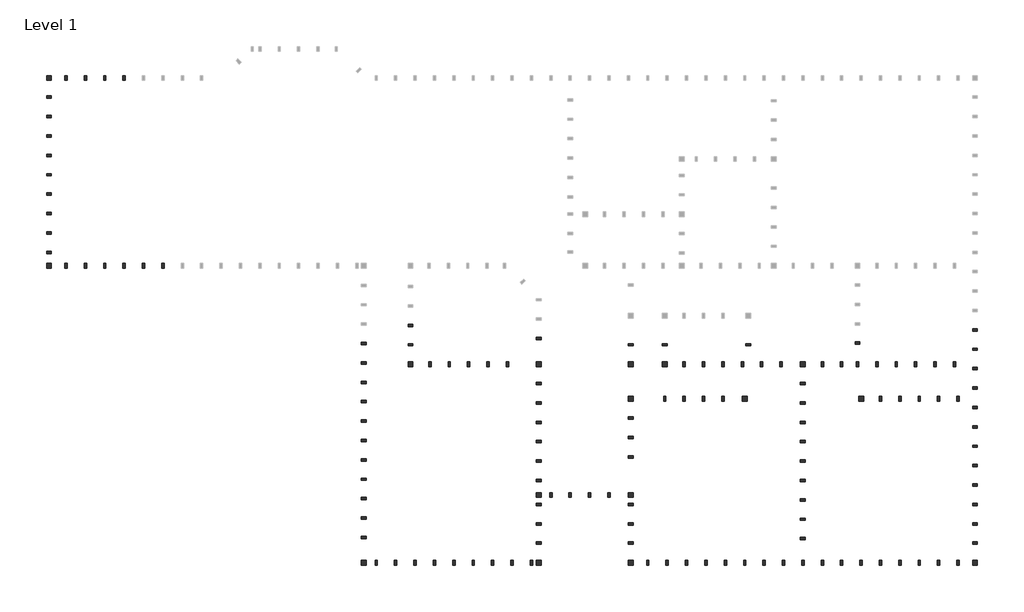
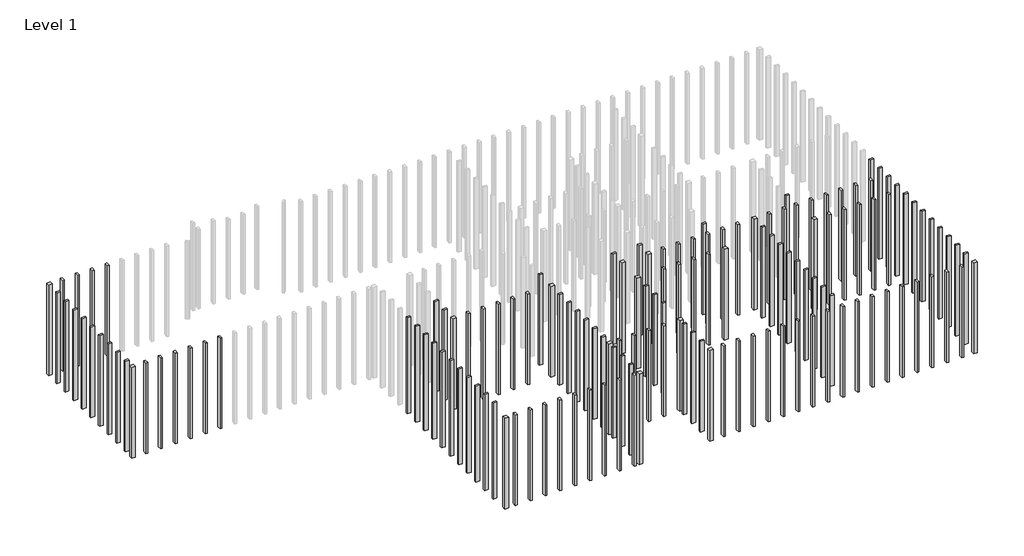
# One storey, part 1 of 2: 147 columns.
"""IFC4 building model written with IfcOpenShell, lengths in millimetres."""

import ifcopenshell
import ifcopenshell.guid

model = None  # the IFC model being written
_history = None  # IfcOwnerHistory: only IFC2X3 demands one
_inside = {}  # id of a spatial element -> (the spatial element, [elements in it])
_under = {}  # id of a project, library or spatial element -> (it, [spatial elements below it])
_declared = {}  # id of a project -> (the project, [libraries it declares])
_typed = {}  # id of a type object -> (the type object, [elements of that type])
_made_of = {}  # id of a material, layer set ... -> (it, [elements and type objects made of it])


def new_model(schema):
    """Start an empty IFC model of exactly this schema.

    Asked for "IFC4X3", IfcOpenShell would pick the latest addendum, in which some entities
    have other attributes; the version numbers below select the first issue.
    IFC2X3 requires an IfcOwnerHistory on every rooted entity: one is made here for all.
    """
    global model, _history
    if schema == "IFC4X3":
        model = ifcopenshell.file(schema_version=(4, 3, 0, 0))
    else:
        model = ifcopenshell.file(schema=schema)
    _inside.clear()
    _under.clear()
    _declared.clear()
    _typed.clear()
    _made_of.clear()
    _history = None
    if model.schema == "IFC2X3":
        org = make("IfcOrganization", Name="unknown")
        user = make(
            "IfcPersonAndOrganization",
            ThePerson=make("IfcPerson", FamilyName="unknown"),
            TheOrganization=org,
        )
        app = make(
            "IfcApplication",
            ApplicationDeveloper=org,
            Version="unknown",
            ApplicationFullName="unknown",
            ApplicationIdentifier="unknown",
        )
        _history = make(
            "IfcOwnerHistory",
            OwningUser=user,
            OwningApplication=app,
            ChangeAction="ADDED",
            CreationDate=0,
        )
    return model


def make(cls, **values):
    """One entity of the class cls with the attributes given. An attribute that is None is left unset."""
    return model.create_entity(
        cls, **{name: value for name, value in values.items() if value is not None}
    )


def rooted(cls, **values):
    """An entity with a GlobalId (a new one), such as an element, a storey or a relation."""
    return make(cls, GlobalId=ifcopenshell.guid.new(), OwnerHistory=_history, **values)


def si_unit(unit_type, name, prefix=None):
    """IfcSIUnit, for example si_unit("LENGTHUNIT", "METRE", prefix="MILLI")."""
    return make("IfcSIUnit", UnitType=unit_type, Prefix=prefix, Name=name)


def assignment(units):
    """IfcUnitAssignment: the units of a project."""
    return None if units is None else make("IfcUnitAssignment", Units=units)


def point(xyz):
    """IfcCartesianPoint."""
    return None if xyz is None else make("IfcCartesianPoint", Coordinates=xyz)


def direction(xyz):
    """IfcDirection."""
    return None if xyz is None else make("IfcDirection", DirectionRatios=xyz)


def frame(location, z_axis=None, x_axis=None):
    """IfcAxis2Placement3D, a coordinate frame: its origin and axes. An axis left out is left unset."""
    return make(
        "IfcAxis2Placement3D",
        Location=point(location),
        Axis=direction(z_axis),
        RefDirection=direction(x_axis),
    )


def origin():
    """The frame at (0, 0, 0) with its axes left unset."""
    return frame((0.0, 0.0, 0.0))


def origin_with_axes():
    """The frame at (0, 0, 0) with the z axis (0, 0, 1) and the x axis (1, 0, 0) written out."""
    return frame((0.0, 0.0, 0.0), z_axis=(0.0, 0.0, 1.0), x_axis=(1.0, 0.0, 0.0))


def place(relative_to, where):
    """IfcLocalPlacement: puts the frame where relative to a parent placement (None: the world)."""
    return make(
        "IfcLocalPlacement", PlacementRelTo=relative_to, RelativePlacement=where
    )


def context(
    kind, dimensions, precision=None, world=None, true_north=None, identifier=None
):
    """IfcGeometricRepresentationContext, for example the 3D "Model" context."""
    return make(
        "IfcGeometricRepresentationContext",
        ContextIdentifier=identifier,
        ContextType=kind,
        CoordinateSpaceDimension=dimensions,
        Precision=precision,
        WorldCoordinateSystem=world,
        TrueNorth=true_north,
    )


def project(units=None, contexts=None):
    """IfcProject with its units and contexts."""
    return rooted(
        "IfcProject",
        Name="project",
        RepresentationContexts=contexts,
        UnitsInContext=assignment(units),
    )


def spatial(cls, under=None, at=None, **own):
    """A site, building, storey or space (cls), placed at a placement, below another one or the project."""
    s = rooted(cls, ObjectPlacement=at, **own)
    if under is not None:
        _under.setdefault(under.id(), (under, []))[1].append(s)
    return s


def polyline(points):
    """IfcPolyline through the points."""
    return make("IfcPolyline", Points=[point(p) for p in points])


def outline(outer, holes=None, kind="AREA"):
    """IfcArbitraryClosedProfileDef: a profile drawn as a closed curve; with holes, ...WithVoids."""
    if holes is None:
        return make("IfcArbitraryClosedProfileDef", ProfileType=kind, OuterCurve=outer)
    return make(
        "IfcArbitraryProfileDefWithVoids",
        ProfileType=kind,
        OuterCurve=outer,
        InnerCurves=holes,
    )


def extrude(swept, where, along, depth):
    """IfcExtrudedAreaSolid: the profile swept, set in the frame where, extruded along a direction by depth."""
    return make(
        "IfcExtrudedAreaSolid",
        SweptArea=swept,
        Position=where,
        ExtrudedDirection=direction(along),
        Depth=depth,
    )


def shape(context_of_items, identifier, shape_type, items):
    """IfcShapeRepresentation: the items that make up one representation, for example the "Body"."""
    return make(
        "IfcShapeRepresentation",
        ContextOfItems=context_of_items,
        RepresentationIdentifier=identifier,
        RepresentationType=shape_type,
        Items=items,
    )


def source(mapping_origin, context_of_items, identifier, shape_type, items):
    """IfcRepresentationMap: a shape defined once, which mapped items show again and again."""
    return make(
        "IfcRepresentationMap",
        MappingOrigin=mapping_origin,
        MappedRepresentation=shape(context_of_items, identifier, shape_type, items),
    )


def transform(
    local_origin,
    x_axis=None,
    y_axis=None,
    z_axis=None,
    scale=None,
    scale2=None,
    scale3=None,
    uniform=True,
):
    """IfcCartesianTransformationOperator3D, or its non-uniform kind. x_axis, y_axis, z_axis: its Axis1, 2, 3."""
    if uniform:
        return make(
            "IfcCartesianTransformationOperator3D",
            Axis1=direction(x_axis),
            Axis2=direction(y_axis),
            LocalOrigin=point(local_origin),
            Scale=scale,
            Axis3=direction(z_axis),
        )
    return make(
        "IfcCartesianTransformationOperator3DnonUniform",
        Axis1=direction(x_axis),
        Axis2=direction(y_axis),
        LocalOrigin=point(local_origin),
        Scale=scale,
        Axis3=direction(z_axis),
        Scale2=scale2,
        Scale3=scale3,
    )


def mapped(mapping_source, mapping_target):
    """IfcMappedItem: shows the shape of a source again, moved by a transform."""
    return make(
        "IfcMappedItem", MappingSource=mapping_source, MappingTarget=mapping_target
    )


def made_of(thing, what):
    """Note that an element or type object is made of a material, layer set ...; save() writes the relation."""
    if what is not None:
        _made_of.setdefault(what.id(), (what, []))[1].append(thing)
    return thing


def element(
    cls,
    number,
    at=None,
    inside=None,
    cuts=None,
    type_object=None,
    material=None,
    context=None,
    identifier="Body",
    shape_type=None,
    held_by="IfcProductDefinitionShape",
    body=None,
    shapes=None,
    **own,
):
    """One element of the class cls, such as IfcWall. Its Tag is "e" and its number.

    at: its placement. inside: the storey or other place that contains it. cuts: it is an
    opening in that element (IfcRelVoidsElement). A single representation is given by context,
    identifier, shape_type and body (its items); several are given by shapes. held_by: the class
    of the entity that holds the representations. save() writes the other relations.
    """
    e = rooted(cls, Tag="e%d" % number, ObjectPlacement=at, **own)
    if body is not None:
        shapes = [shape(context, identifier, shape_type, body)]
    if shapes is not None:
        e.Representation = make(held_by, Representations=shapes)
    if inside is not None:
        _inside.setdefault(inside.id(), (inside, []))[1].append(e)
    if cuts is not None:
        rooted(
            "IfcRelVoidsElement", RelatingBuildingElement=cuts, RelatedOpeningElement=e
        )
    if type_object is not None:
        _typed.setdefault(type_object.id(), (type_object, []))[1].append(e)
    return made_of(e, material)


def aggregate(whole, parts):
    """IfcRelAggregates: a whole, such as a stair, and the parts it consists of."""
    return rooted("IfcRelAggregates", RelatingObject=whole, RelatedObjects=parts)


def save(model, path):
    """Write the relations noted so far, then the file.

    IfcRelAggregates (storeys below a building ...), IfcRelContainedInSpatialStructure (elements
    in a storey), IfcRelDefinesByType, IfcRelAssociatesMaterial and IfcRelDeclares: one each for
    every whole, place, type object, material and project.
    """
    for whole, parts in _under.values():
        aggregate(whole, parts)
    for where, things in _inside.values():
        rooted(
            "IfcRelContainedInSpatialStructure",
            RelatedElements=things,
            RelatingStructure=where,
        )
    for kind, things in _typed.values():
        rooted("IfcRelDefinesByType", RelatedObjects=things, RelatingType=kind)
    for what, things in _made_of.values():
        rooted("IfcRelAssociatesMaterial", RelatedObjects=things, RelatingMaterial=what)
    for by, libraries in _declared.values():
        rooted("IfcRelDeclares", RelatingContext=by, RelatedDefinitions=libraries)
    model.write(path)


def timber_column_65e54e3c(model_context):
    return source(origin(), model_context, "Body", "SweptSolid", [
        extrude(outline(polyline([(25.4, 50.8), (25.4, -50.8), (-25.4, -50.8), (-25.4, 50.8), (25.4, 50.8)])), frame((0.0, 0.0, 50.8), z_axis=(0.0, 0.0, 1.0), x_axis=(1.0, 0.0, 0.0)), (0.0, 0.0, 1.0), 2616.2),
    ])


def timber_column_b7e6a7b9(model_context):
    return source(origin(), model_context, "Body", "SweptSolid", [
        extrude(outline(polyline([(50.8, 50.8), (50.8, -50.8), (-50.8, -50.8), (-50.8, 50.8), (50.8, 50.8)])), frame((0.0, 0.0, 50.8), z_axis=(0.0, 0.0, 1.0), x_axis=(1.0, 0.0, 0.0)), (0.0, 0.0, 1.0), 2616.2),
    ])


def timber_column_c014de30(model_context):
    return source(origin(), model_context, "Body", "SweptSolid", [
        extrude(outline(polyline([(25.4, -50.8), (-25.4, -50.8), (-25.4, 50.8), (25.4, 50.8), (25.4, -50.8)])), frame((0.0, 0.0, 50.8), z_axis=(0.0, 0.0, 1.0), x_axis=(1.0, 0.0, 0.0)), (0.0, 0.0, 1.0), 2616.2),
    ])


def timber_column_7e99ce9a(model_context):
    return source(origin(), model_context, "Body", "SweptSolid", [
        extrude(outline(polyline([(25.4, 50.8), (25.4, -50.8), (-25.4, -50.8), (-25.4, 50.8), (25.4, 50.8)])), origin_with_axes(), (0.0, 0.0, 1.0), 2768.6),
    ])


model = new_model("IFC4")

# Units and contexts
model_context = context("Model", 3, world=origin())
ifc_project = project(units=[si_unit("LENGTHUNIT", "METRE", prefix="MILLI")], contexts=[model_context])

# Site, building, storey
site = spatial("IfcSite", under=ifc_project)
building = spatial("IfcBuilding", under=site)
storey = spatial("IfcBuildingStorey", under=building, Name="Level 1", Elevation=0.0)

# Columns
placement = place(None, origin())
timber_column_shape = timber_column_65e54e3c(model_context)
element("IfcColumn", 1, ObjectType="Timber-Column", at=placement, inside=storey, context=model_context, shape_type="MappedRepresentation", body=[
    mapped(timber_column_shape, transform((-17394.814829, 5156.9284114, 0.0), x_axis=(1.0, 0.0, 0.0), y_axis=(0.0, 1.0, 0.0), z_axis=(0.0, 0.0, 1.0))),
])
element("IfcColumn", 2, ObjectType="Timber-Column", at=placement, inside=storey, context=model_context, shape_type="MappedRepresentation", body=[
    mapped(timber_column_shape, transform((-16988.414829, 5156.9284114, 0.0), x_axis=(1.0, 0.0, 0.0), y_axis=(0.0, 1.0, 0.0), z_axis=(0.0, 0.0, 1.0))),
])
element("IfcColumn", 3, ObjectType="Timber-Column", at=placement, inside=storey, context=model_context, shape_type="MappedRepresentation", body=[
    mapped(timber_column_shape, transform((-16582.014829, 5156.9284114, 0.0), x_axis=(1.0, 0.0, 0.0), y_axis=(0.0, 1.0, 0.0), z_axis=(0.0, 0.0, 1.0))),
])
element("IfcColumn", 4, ObjectType="Timber-Column", at=placement, inside=storey, context=model_context, shape_type="MappedRepresentation", body=[
    mapped(timber_column_shape, transform((-16175.614829, 5156.9284114, 0.0), x_axis=(1.0, 0.0, 0.0), y_axis=(0.0, 1.0, 0.0), z_axis=(0.0, 0.0, 1.0))),
])
element("IfcColumn", 5, ObjectType="Timber-Column", at=placement, inside=storey, context=model_context, shape_type="MappedRepresentation", body=[
    mapped(timber_column_shape, transform((1299.585171, -5003.0715886, 0.0), x_axis=(1.0, 0.0, 0.0), y_axis=(0.0, 1.0, 0.0), z_axis=(0.0, 0.0, 1.0))),
])
element("IfcColumn", 6, ObjectType="Timber-Column", at=placement, inside=storey, context=model_context, shape_type="MappedRepresentation", body=[
    mapped(timber_column_shape, transform((893.185171, -5003.0715886, 0.0), x_axis=(1.0, 0.0, 0.0), y_axis=(0.0, 1.0, 0.0), z_axis=(0.0, 0.0, 1.0))),
])
element("IfcColumn", 7, ObjectType="Timber-Column", at=placement, inside=storey, context=model_context, shape_type="MappedRepresentation", body=[
    mapped(timber_column_shape, transform((486.785171, -5003.0715886, 0.0), x_axis=(1.0, 0.0, 0.0), y_axis=(0.0, 1.0, 0.0), z_axis=(0.0, 0.0, 1.0))),
])
element("IfcColumn", 8, ObjectType="Timber-Column", at=placement, inside=storey, context=model_context, shape_type="MappedRepresentation", body=[
    mapped(timber_column_shape, transform((80.385171, -5003.0715886, 0.0), x_axis=(1.0, 0.0, 0.0), y_axis=(0.0, 1.0, 0.0), z_axis=(0.0, 0.0, 1.0))),
])
element("IfcColumn", 9, ObjectType="Timber-Column", at=placement, inside=storey, context=model_context, shape_type="MappedRepresentation", body=[
    mapped(timber_column_shape, transform((-326.014829, -5003.0715886, 0.0), x_axis=(1.0, 0.0, 0.0), y_axis=(0.0, 1.0, 0.0), z_axis=(0.0, 0.0, 1.0))),
])
element("IfcColumn", 10, ObjectType="Timber-Column", at=placement, inside=storey, context=model_context, shape_type="MappedRepresentation", body=[
    mapped(timber_column_shape, transform((-732.414829, -5003.0715886, 0.0), x_axis=(1.0, 0.0, 0.0), y_axis=(0.0, 1.0, 0.0), z_axis=(0.0, 0.0, 1.0))),
])
element("IfcColumn", 11, ObjectType="Timber-Column", at=placement, inside=storey, context=model_context, shape_type="MappedRepresentation", body=[
    mapped(timber_column_shape, transform((-1138.814829, -5003.0715886, 0.0), x_axis=(1.0, 0.0, 0.0), y_axis=(0.0, 1.0, 0.0), z_axis=(0.0, 0.0, 1.0))),
])
element("IfcColumn", 12, ObjectType="Timber-Column", at=placement, inside=storey, context=model_context, shape_type="MappedRepresentation", body=[
    mapped(timber_column_shape, transform((-1545.214829, -5003.0715886, 0.0), x_axis=(1.0, 0.0, 0.0), y_axis=(0.0, 1.0, 0.0), z_axis=(0.0, 0.0, 1.0))),
])
element("IfcColumn", 13, ObjectType="Timber-Column", at=placement, inside=storey, context=model_context, shape_type="MappedRepresentation", body=[
    mapped(timber_column_shape, transform((-1951.614829, -5003.0715886, 0.0), x_axis=(1.0, 0.0, 0.0), y_axis=(0.0, 1.0, 0.0), z_axis=(0.0, 0.0, 1.0))),
])
element("IfcColumn", 14, ObjectType="Timber-Column", at=placement, inside=storey, context=model_context, shape_type="MappedRepresentation", body=[
    mapped(timber_column_shape, transform((-2358.014829, -5003.0715886, 0.0), x_axis=(1.0, 0.0, 0.0), y_axis=(0.0, 1.0, 0.0), z_axis=(0.0, 0.0, 1.0))),
])
element("IfcColumn", 15, ObjectType="Timber-Column", at=placement, inside=storey, context=model_context, shape_type="MappedRepresentation", body=[
    mapped(timber_column_shape, transform((-2764.414829, -5003.0715886, 0.0), x_axis=(1.0, 0.0, 0.0), y_axis=(0.0, 1.0, 0.0), z_axis=(0.0, 0.0, 1.0))),
])
element("IfcColumn", 16, ObjectType="Timber-Column", at=placement, inside=storey, context=model_context, shape_type="MappedRepresentation", body=[
    mapped(timber_column_shape, transform((-3170.814829, -5003.0715886, 0.0), x_axis=(1.0, 0.0, 0.0), y_axis=(0.0, 1.0, 0.0), z_axis=(0.0, 0.0, 1.0))),
])
element("IfcColumn", 17, ObjectType="Timber-Column", at=placement, inside=storey, context=model_context, shape_type="MappedRepresentation", body=[
    mapped(timber_column_shape, transform((-3577.214829, -5003.0715886, 0.0), x_axis=(1.0, 0.0, 0.0), y_axis=(0.0, 1.0, 0.0), z_axis=(0.0, 0.0, 1.0))),
])
element("IfcColumn", 18, ObjectType="Timber-Column", at=placement, inside=storey, context=model_context, shape_type="MappedRepresentation", body=[
    mapped(timber_column_shape, transform((-3983.614829, -5003.0715886, 0.0), x_axis=(1.0, 0.0, 0.0), y_axis=(0.0, 1.0, 0.0), z_axis=(0.0, 0.0, 1.0))),
])
element("IfcColumn", 19, ObjectType="Timber-Column", at=placement, inside=storey, context=model_context, shape_type="MappedRepresentation", body=[
    mapped(timber_column_shape, transform((-4390.014829, -5003.0715886, 0.0), x_axis=(1.0, 0.0, 0.0), y_axis=(0.0, 1.0, 0.0), z_axis=(0.0, 0.0, 1.0))),
])
element("IfcColumn", 20, ObjectType="Timber-Column", at=placement, inside=storey, context=model_context, shape_type="MappedRepresentation", body=[
    mapped(timber_column_shape, transform((-4796.414829, -5003.0715886, 0.0), x_axis=(1.0, 0.0, 0.0), y_axis=(0.0, 1.0, 0.0), z_axis=(0.0, 0.0, 1.0))),
])
element("IfcColumn", 21, ObjectType="Timber-Column", at=placement, inside=storey, context=model_context, shape_type="MappedRepresentation", body=[
    mapped(timber_column_shape, transform((-5202.814829, -5003.0715886, 0.0), x_axis=(1.0, 0.0, 0.0), y_axis=(0.0, 1.0, 0.0), z_axis=(0.0, 0.0, 1.0))),
])
element("IfcColumn", 22, ObjectType="Timber-Column", at=placement, inside=storey, context=model_context, shape_type="MappedRepresentation", body=[
    mapped(timber_column_shape, transform((-6015.614829, -3580.6715886, 0.0), x_axis=(1.0, 0.0, 0.0), y_axis=(0.0, 1.0, 0.0), z_axis=(0.0, 0.0, 1.0))),
])
element("IfcColumn", 23, ObjectType="Timber-Column", at=placement, inside=storey, context=model_context, shape_type="MappedRepresentation", body=[
    mapped(timber_column_shape, transform((-6422.014829, -3580.6715886, 0.0), x_axis=(1.0, 0.0, 0.0), y_axis=(0.0, 1.0, 0.0), z_axis=(0.0, 0.0, 1.0))),
])
element("IfcColumn", 24, ObjectType="Timber-Column", at=placement, inside=storey, context=model_context, shape_type="MappedRepresentation", body=[
    mapped(timber_column_shape, transform((-6828.414829, -3580.6715886, 0.0), x_axis=(1.0, 0.0, 0.0), y_axis=(0.0, 1.0, 0.0), z_axis=(0.0, 0.0, 1.0))),
])
element("IfcColumn", 25, ObjectType="Timber-Column", at=placement, inside=storey, context=model_context, shape_type="MappedRepresentation", body=[
    mapped(timber_column_shape, transform((-7234.814829, -3580.6715886, 0.0), x_axis=(1.0, 0.0, 0.0), y_axis=(0.0, 1.0, 0.0), z_axis=(0.0, 0.0, 1.0))),
])
element("IfcColumn", 26, ObjectType="Timber-Column", at=placement, inside=storey, context=model_context, shape_type="MappedRepresentation", body=[
    mapped(timber_column_shape, transform((-7641.214829, -5003.0715886, 0.0), x_axis=(1.0, 0.0, 0.0), y_axis=(0.0, 1.0, 0.0), z_axis=(0.0, 0.0, 1.0))),
])
element("IfcColumn", 27, ObjectType="Timber-Column", at=placement, inside=storey, context=model_context, shape_type="MappedRepresentation", body=[
    mapped(timber_column_shape, transform((-8047.614829, -5003.0715886, 0.0), x_axis=(1.0, 0.0, 0.0), y_axis=(0.0, 1.0, 0.0), z_axis=(0.0, 0.0, 1.0))),
])
element("IfcColumn", 28, ObjectType="Timber-Column", at=placement, inside=storey, context=model_context, shape_type="MappedRepresentation", body=[
    mapped(timber_column_shape, transform((-8454.014829, -5003.0715886, 0.0), x_axis=(1.0, 0.0, 0.0), y_axis=(0.0, 1.0, 0.0), z_axis=(0.0, 0.0, 1.0))),
])
element("IfcColumn", 29, ObjectType="Timber-Column", at=placement, inside=storey, context=model_context, shape_type="MappedRepresentation", body=[
    mapped(timber_column_shape, transform((-8860.414829, -5003.0715886, 0.0), x_axis=(1.0, 0.0, 0.0), y_axis=(0.0, 1.0, 0.0), z_axis=(0.0, 0.0, 1.0))),
])
element("IfcColumn", 30, ObjectType="Timber-Column", at=placement, inside=storey, context=model_context, shape_type="MappedRepresentation", body=[
    mapped(timber_column_shape, transform((-9266.814829, -5003.0715886, 0.0), x_axis=(1.0, 0.0, 0.0), y_axis=(0.0, 1.0, 0.0), z_axis=(0.0, 0.0, 1.0))),
])
element("IfcColumn", 31, ObjectType="Timber-Column", at=placement, inside=storey, context=model_context, shape_type="MappedRepresentation", body=[
    mapped(timber_column_shape, transform((-9673.214829, -5003.0715886, 0.0), x_axis=(1.0, 0.0, 0.0), y_axis=(0.0, 1.0, 0.0), z_axis=(0.0, 0.0, 1.0))),
])
element("IfcColumn", 32, ObjectType="Timber-Column", at=placement, inside=storey, context=model_context, shape_type="MappedRepresentation", body=[
    mapped(timber_column_shape, transform((-10079.614829, -5003.0715886, 0.0), x_axis=(1.0, 0.0, 0.0), y_axis=(0.0, 1.0, 0.0), z_axis=(0.0, 0.0, 1.0))),
])
element("IfcColumn", 33, ObjectType="Timber-Column", at=placement, inside=storey, context=model_context, shape_type="MappedRepresentation", body=[
    mapped(timber_column_shape, transform((-10486.014829, -5003.0715886, 0.0), x_axis=(1.0, 0.0, 0.0), y_axis=(0.0, 1.0, 0.0), z_axis=(0.0, 0.0, 1.0))),
])
element("IfcColumn", 34, ObjectType="Timber-Column", at=placement, inside=storey, context=model_context, shape_type="MappedRepresentation", body=[
    mapped(timber_column_shape, transform((-10892.414829, -5003.0715886, 0.0), x_axis=(1.0, 0.0, 0.0), y_axis=(0.0, 1.0, 0.0), z_axis=(0.0, 0.0, 1.0))),
])
element("IfcColumn", 35, ObjectType="Timber-Column", at=placement, inside=storey, context=model_context, shape_type="MappedRepresentation", body=[
    mapped(timber_column_shape, transform((-15362.814829, 1226.2784114, 0.0), x_axis=(1.0, 0.0, 0.0), y_axis=(0.0, 1.0, 0.0), z_axis=(0.0, 0.0, 1.0))),
])
element("IfcColumn", 36, ObjectType="Timber-Column", at=placement, inside=storey, context=model_context, shape_type="MappedRepresentation", body=[
    mapped(timber_column_shape, transform((-15769.214829, 1226.2784114, 0.0), x_axis=(1.0, 0.0, 0.0), y_axis=(0.0, 1.0, 0.0), z_axis=(0.0, 0.0, 1.0))),
])
element("IfcColumn", 37, ObjectType="Timber-Column", at=placement, inside=storey, context=model_context, shape_type="MappedRepresentation", body=[
    mapped(timber_column_shape, transform((-16175.614829, 1226.2784114, 0.0), x_axis=(1.0, 0.0, 0.0), y_axis=(0.0, 1.0, 0.0), z_axis=(0.0, 0.0, 1.0))),
])
element("IfcColumn", 38, ObjectType="Timber-Column", at=placement, inside=storey, context=model_context, shape_type="MappedRepresentation", body=[
    mapped(timber_column_shape, transform((-16582.014829, 1226.2784114, 0.0), x_axis=(1.0, 0.0, 0.0), y_axis=(0.0, 1.0, 0.0), z_axis=(0.0, 0.0, 1.0))),
])
element("IfcColumn", 39, ObjectType="Timber-Column", at=placement, inside=storey, context=model_context, shape_type="MappedRepresentation", body=[
    mapped(timber_column_shape, transform((-16988.414829, 1226.2784114, 0.0), x_axis=(1.0, 0.0, 0.0), y_axis=(0.0, 1.0, 0.0), z_axis=(0.0, 0.0, 1.0))),
])
element("IfcColumn", 40, ObjectType="Timber-Column", at=placement, inside=storey, context=model_context, shape_type="MappedRepresentation", body=[
    mapped(timber_column_shape, transform((-17394.814829, 1226.2784114, 0.0), x_axis=(1.0, 0.0, 0.0), y_axis=(0.0, 1.0, 0.0), z_axis=(0.0, 0.0, 1.0))),
])
element("IfcColumn", 41, ObjectType="Timber-Column", at=placement, inside=storey, context=model_context, shape_type="MappedRepresentation", body=[
    mapped(timber_column_shape, transform((-17750.414829, 4756.8784114, 0.0), x_axis=(0.0, 1.0, 0.0), y_axis=(-1.0, 0.0, 0.0), z_axis=(0.0, 0.0, 1.0))),
])
element("IfcColumn", 42, ObjectType="Timber-Column", at=placement, inside=storey, context=model_context, shape_type="MappedRepresentation", body=[
    mapped(timber_column_shape, transform((-17750.414829, 4350.4784114, 0.0), x_axis=(0.0, 1.0, 0.0), y_axis=(-1.0, 0.0, 0.0), z_axis=(0.0, 0.0, 1.0))),
])
element("IfcColumn", 43, ObjectType="Timber-Column", at=placement, inside=storey, context=model_context, shape_type="MappedRepresentation", body=[
    mapped(timber_column_shape, transform((-17750.414829, 3944.0784114, 0.0), x_axis=(0.0, 1.0, 0.0), y_axis=(-1.0, 0.0, 0.0), z_axis=(0.0, 0.0, 1.0))),
])
element("IfcColumn", 44, ObjectType="Timber-Column", at=placement, inside=storey, context=model_context, shape_type="MappedRepresentation", body=[
    mapped(timber_column_shape, transform((-17750.414829, 3537.6784114, 0.0), x_axis=(0.0, 1.0, 0.0), y_axis=(-1.0, 0.0, 0.0), z_axis=(0.0, 0.0, 1.0))),
])
element("IfcColumn", 45, ObjectType="Timber-Column", at=placement, inside=storey, context=model_context, shape_type="MappedRepresentation", body=[
    mapped(timber_column_shape, transform((-17750.414829, 3131.2784114, 0.0), x_axis=(0.0, 1.0, 0.0), y_axis=(-1.0, 0.0, 0.0), z_axis=(0.0, 0.0, 1.0))),
])
element("IfcColumn", 46, ObjectType="Timber-Column", at=placement, inside=storey, context=model_context, shape_type="MappedRepresentation", body=[
    mapped(timber_column_shape, transform((-17750.414829, 2724.8784114, 0.0), x_axis=(0.0, 1.0, 0.0), y_axis=(-1.0, 0.0, 0.0), z_axis=(0.0, 0.0, 1.0))),
])
element("IfcColumn", 47, ObjectType="Timber-Column", at=placement, inside=storey, context=model_context, shape_type="MappedRepresentation", body=[
    mapped(timber_column_shape, transform((-17750.414829, 2318.4784114, 0.0), x_axis=(0.0, 1.0, 0.0), y_axis=(-1.0, 0.0, 0.0), z_axis=(0.0, 0.0, 1.0))),
])
element("IfcColumn", 48, ObjectType="Timber-Column", at=placement, inside=storey, context=model_context, shape_type="MappedRepresentation", body=[
    mapped(timber_column_shape, transform((-17750.414829, 1912.0784114, 0.0), x_axis=(0.0, 1.0, 0.0), y_axis=(-1.0, 0.0, 0.0), z_axis=(0.0, 0.0, 1.0))),
])
element("IfcColumn", 49, ObjectType="Timber-Column", at=placement, inside=storey, context=model_context, shape_type="MappedRepresentation", body=[
    mapped(timber_column_shape, transform((-17750.414829, 1505.6784114, 0.0), x_axis=(0.0, 1.0, 0.0), y_axis=(-1.0, 0.0, 0.0), z_axis=(0.0, 0.0, 1.0))),
])
element("IfcColumn", 50, ObjectType="Timber-Column", at=placement, inside=storey, context=model_context, shape_type="MappedRepresentation", body=[
    mapped(timber_column_shape, transform((-7488.814829, -301.7056866, 0.0), x_axis=(0.0, 1.0, 0.0), y_axis=(-1.0, 0.0, 0.0), z_axis=(0.0, 0.0, 1.0))),
])
element("IfcColumn", 51, ObjectType="Timber-Column", at=placement, inside=storey, context=model_context, shape_type="MappedRepresentation", body=[
    mapped(timber_column_shape, transform((-9768.464829, -837.4715886, 0.0), x_axis=(1.0, 0.0, 0.0), y_axis=(0.0, 1.0, 0.0), z_axis=(0.0, 0.0, 1.0))),
])
element("IfcColumn", 52, ObjectType="Timber-Column", at=placement, inside=storey, context=model_context, shape_type="MappedRepresentation", body=[
    mapped(timber_column_shape, transform((-9362.064829, -837.4715886, 0.0), x_axis=(1.0, 0.0, 0.0), y_axis=(0.0, 1.0, 0.0), z_axis=(0.0, 0.0, 1.0))),
])
element("IfcColumn", 53, ObjectType="Timber-Column", at=placement, inside=storey, context=model_context, shape_type="MappedRepresentation", body=[
    mapped(timber_column_shape, transform((-8955.664829, -837.4715886, 0.0), x_axis=(1.0, 0.0, 0.0), y_axis=(0.0, 1.0, 0.0), z_axis=(0.0, 0.0, 1.0))),
])
element("IfcColumn", 54, ObjectType="Timber-Column", at=placement, inside=storey, context=model_context, shape_type="MappedRepresentation", body=[
    mapped(timber_column_shape, transform((-8549.264829, -837.4715886, 0.0), x_axis=(1.0, 0.0, 0.0), y_axis=(0.0, 1.0, 0.0), z_axis=(0.0, 0.0, 1.0))),
])
element("IfcColumn", 55, ObjectType="Timber-Column", at=placement, inside=storey, context=model_context, shape_type="MappedRepresentation", body=[
    mapped(timber_column_shape, transform((-8142.864829, -837.4715886, 0.0), x_axis=(1.0, 0.0, 0.0), y_axis=(0.0, 1.0, 0.0), z_axis=(0.0, 0.0, 1.0))),
])
element("IfcColumn", 56, ObjectType="Timber-Column", at=placement, inside=storey, context=model_context, shape_type="MappedRepresentation", body=[
    mapped(timber_column_shape, transform((-7488.814829, -1243.8715886, 0.0), x_axis=(0.0, 1.0, 0.0), y_axis=(-1.0, 0.0, 0.0), z_axis=(0.0, 0.0, 1.0))),
])
element("IfcColumn", 57, ObjectType="Timber-Column", at=placement, inside=storey, context=model_context, shape_type="MappedRepresentation", body=[
    mapped(timber_column_shape, transform((-7488.814829, -1650.2715886, 0.0), x_axis=(0.0, 1.0, 0.0), y_axis=(-1.0, 0.0, 0.0), z_axis=(0.0, 0.0, 1.0))),
])
element("IfcColumn", 58, ObjectType="Timber-Column", at=placement, inside=storey, context=model_context, shape_type="MappedRepresentation", body=[
    mapped(timber_column_shape, transform((-7488.814829, -2056.6715886, 0.0), x_axis=(0.0, 1.0, 0.0), y_axis=(-1.0, 0.0, 0.0), z_axis=(0.0, 0.0, 1.0))),
])
element("IfcColumn", 59, ObjectType="Timber-Column", at=placement, inside=storey, context=model_context, shape_type="MappedRepresentation", body=[
    mapped(timber_column_shape, transform((-7488.814829, -2463.0715886, 0.0), x_axis=(0.0, 1.0, 0.0), y_axis=(-1.0, 0.0, 0.0), z_axis=(0.0, 0.0, 1.0))),
])
element("IfcColumn", 60, ObjectType="Timber-Column", at=placement, inside=storey, context=model_context, shape_type="MappedRepresentation", body=[
    mapped(timber_column_shape, transform((-7488.814829, -2869.4715886, 0.0), x_axis=(0.0, 1.0, 0.0), y_axis=(-1.0, 0.0, 0.0), z_axis=(0.0, 0.0, 1.0))),
])
element("IfcColumn", 61, ObjectType="Timber-Column", at=placement, inside=storey, context=model_context, shape_type="MappedRepresentation", body=[
    mapped(timber_column_shape, transform((-7488.814829, -3275.8715886, 0.0), x_axis=(0.0, 1.0, 0.0), y_axis=(-1.0, 0.0, 0.0), z_axis=(0.0, 0.0, 1.0))),
])
element("IfcColumn", 62, ObjectType="Timber-Column", at=placement, inside=storey, context=model_context, shape_type="MappedRepresentation", body=[
    mapped(timber_column_shape, transform((-10175.1225949, -431.0715886, 0.0), x_axis=(0.0, 1.0, 0.0), y_axis=(-1.0, 0.0, 0.0), z_axis=(0.0, 0.0, 1.0))),
])
element("IfcColumn", 63, ObjectType="Timber-Column", at=placement, inside=storey, context=model_context, shape_type="MappedRepresentation", body=[
    mapped(timber_column_shape, transform((-10175.1225949, -24.6715886, 0.0), x_axis=(0.0, 1.0, 0.0), y_axis=(-1.0, 0.0, 0.0), z_axis=(0.0, 0.0, 1.0))),
])
element("IfcColumn", 64, ObjectType="Timber-Column", at=placement, inside=storey, context=model_context, shape_type="MappedRepresentation", body=[
    mapped(timber_column_shape, transform((-5558.414829, -431.0715886, 0.0), x_axis=(0.0, 1.0, 0.0), y_axis=(-1.0, 0.0, 0.0), z_axis=(0.0, 0.0, 1.0))),
])
element("IfcColumn", 65, ObjectType="Timber-Column", at=placement, inside=storey, context=model_context, shape_type="MappedRepresentation", body=[
    mapped(timber_column_shape, transform((-5558.414829, -1967.7715886, 0.0), x_axis=(0.0, 1.0, 0.0), y_axis=(-1.0, 0.0, 0.0), z_axis=(0.0, 0.0, 1.0))),
])
element("IfcColumn", 66, ObjectType="Timber-Column", at=placement, inside=storey, context=model_context, shape_type="MappedRepresentation", body=[
    mapped(timber_column_shape, transform((-5558.414829, -2374.1715886, 0.0), x_axis=(0.0, 1.0, 0.0), y_axis=(-1.0, 0.0, 0.0), z_axis=(0.0, 0.0, 1.0))),
])
element("IfcColumn", 67, ObjectType="Timber-Column", at=placement, inside=storey, context=model_context, shape_type="MappedRepresentation", body=[
    mapped(timber_column_shape, transform((-5558.414829, -2780.5715886, 0.0), x_axis=(0.0, 1.0, 0.0), y_axis=(-1.0, 0.0, 0.0), z_axis=(0.0, 0.0, 1.0))),
])
element("IfcColumn", 68, ObjectType="Timber-Column", at=placement, inside=storey, context=model_context, shape_type="MappedRepresentation", body=[
    mapped(timber_column_shape, transform((-4847.214829, -1561.3715886, 0.0), x_axis=(-1.0, 0.0, 0.0), y_axis=(0.0, -1.0, 0.0), z_axis=(0.0, 0.0, 1.0))),
])
element("IfcColumn", 69, ObjectType="Timber-Column", at=placement, inside=storey, context=model_context, shape_type="MappedRepresentation", body=[
    mapped(timber_column_shape, transform((-4440.814829, -1561.3715886, 0.0), x_axis=(-1.0, 0.0, 0.0), y_axis=(0.0, -1.0, 0.0), z_axis=(0.0, 0.0, 1.0))),
])
element("IfcColumn", 70, ObjectType="Timber-Column", at=placement, inside=storey, context=model_context, shape_type="MappedRepresentation", body=[
    mapped(timber_column_shape, transform((-4034.414829, -1561.3715886, 0.0), x_axis=(-1.0, 0.0, 0.0), y_axis=(0.0, -1.0, 0.0), z_axis=(0.0, 0.0, 1.0))),
])
element("IfcColumn", 71, ObjectType="Timber-Column", at=placement, inside=storey, context=model_context, shape_type="MappedRepresentation", body=[
    mapped(timber_column_shape, transform((-3628.014829, -1561.3715886, 0.0), x_axis=(-1.0, 0.0, 0.0), y_axis=(0.0, -1.0, 0.0), z_axis=(0.0, 0.0, 1.0))),
])
element("IfcColumn", 72, ObjectType="Timber-Column", at=placement, inside=storey, context=model_context, shape_type="MappedRepresentation", body=[
    mapped(timber_column_shape, transform((-4440.814829, -837.4715886, 0.0), x_axis=(-1.0, 0.0, 0.0), y_axis=(0.0, -1.0, 0.0), z_axis=(0.0, 0.0, 1.0))),
])
element("IfcColumn", 73, ObjectType="Timber-Column", at=placement, inside=storey, context=model_context, shape_type="MappedRepresentation", body=[
    mapped(timber_column_shape, transform((-4034.414829, -837.4715886, 0.0), x_axis=(-1.0, 0.0, 0.0), y_axis=(0.0, -1.0, 0.0), z_axis=(0.0, 0.0, 1.0))),
])
element("IfcColumn", 74, ObjectType="Timber-Column", at=placement, inside=storey, context=model_context, shape_type="MappedRepresentation", body=[
    mapped(timber_column_shape, transform((-3628.014829, -837.4715886, 0.0), x_axis=(-1.0, 0.0, 0.0), y_axis=(0.0, -1.0, 0.0), z_axis=(0.0, 0.0, 1.0))),
])
element("IfcColumn", 75, ObjectType="Timber-Column", at=placement, inside=storey, context=model_context, shape_type="MappedRepresentation", body=[
    mapped(timber_column_shape, transform((-3221.614829, -837.4715886, 0.0), x_axis=(-1.0, 0.0, 0.0), y_axis=(0.0, -1.0, 0.0), z_axis=(0.0, 0.0, 1.0))),
])
element("IfcColumn", 76, ObjectType="Timber-Column", at=placement, inside=storey, context=model_context, shape_type="MappedRepresentation", body=[
    mapped(timber_column_shape, transform((-2815.214829, -837.4715886, 0.0), x_axis=(-1.0, 0.0, 0.0), y_axis=(0.0, -1.0, 0.0), z_axis=(0.0, 0.0, 1.0))),
])
element("IfcColumn", 77, ObjectType="Timber-Column", at=placement, inside=storey, context=model_context, shape_type="MappedRepresentation", body=[
    mapped(timber_column_shape, transform((-2408.814829, -837.4715886, 0.0), x_axis=(-1.0, 0.0, 0.0), y_axis=(0.0, -1.0, 0.0), z_axis=(0.0, 0.0, 1.0))),
])
element("IfcColumn", 78, ObjectType="Timber-Column", at=placement, inside=storey, context=model_context, shape_type="MappedRepresentation", body=[
    mapped(timber_column_shape, transform((-4847.214829, -431.0715886, 0.0), x_axis=(0.0, 1.0, 0.0), y_axis=(-1.0, 0.0, 0.0), z_axis=(0.0, 0.0, 1.0))),
])
element("IfcColumn", 79, ObjectType="Timber-Column", at=placement, inside=storey, context=model_context, shape_type="MappedRepresentation", body=[
    mapped(timber_column_shape, transform((-3094.614829, -431.0715886, 0.0), x_axis=(0.0, 1.0, 0.0), y_axis=(-1.0, 0.0, 0.0), z_axis=(0.0, 0.0, 1.0))),
])
element("IfcColumn", 80, ObjectType="Timber-Column", at=placement, inside=storey, context=model_context, shape_type="MappedRepresentation", body=[
    mapped(timber_column_shape, transform((-1545.214829, -837.4715886, 0.0), x_axis=(-1.0, 0.0, 0.0), y_axis=(0.0, -1.0, 0.0), z_axis=(0.0, 0.0, 1.0))),
])
element("IfcColumn", 81, ObjectType="Timber-Column", at=placement, inside=storey, context=model_context, shape_type="MappedRepresentation", body=[
    mapped(timber_column_shape, transform((-1138.814829, -837.4715886, 0.0), x_axis=(-1.0, 0.0, 0.0), y_axis=(0.0, -1.0, 0.0), z_axis=(0.0, 0.0, 1.0))),
])
element("IfcColumn", 82, ObjectType="Timber-Column", at=placement, inside=storey, context=model_context, shape_type="MappedRepresentation", body=[
    mapped(timber_column_shape, transform((-808.614829, -837.4715886, 0.0), x_axis=(-1.0, 0.0, 0.0), y_axis=(0.0, -1.0, 0.0), z_axis=(0.0, 0.0, 1.0))),
])
element("IfcColumn", 83, ObjectType="Timber-Column", at=placement, inside=storey, context=model_context, shape_type="MappedRepresentation", body=[
    mapped(timber_column_shape, transform((-402.214829, -837.4715886, 0.0), x_axis=(-1.0, 0.0, 0.0), y_axis=(0.0, -1.0, 0.0), z_axis=(0.0, 0.0, 1.0))),
])
element("IfcColumn", 84, ObjectType="Timber-Column", at=placement, inside=storey, context=model_context, shape_type="MappedRepresentation", body=[
    mapped(timber_column_shape, transform((4.185171, -837.4715886, 0.0), x_axis=(-1.0, 0.0, 0.0), y_axis=(0.0, -1.0, 0.0), z_axis=(0.0, 0.0, 1.0))),
])
element("IfcColumn", 85, ObjectType="Timber-Column", at=placement, inside=storey, context=model_context, shape_type="MappedRepresentation", body=[
    mapped(timber_column_shape, transform((410.585171, -837.4715886, 0.0), x_axis=(-1.0, 0.0, 0.0), y_axis=(0.0, -1.0, 0.0), z_axis=(0.0, 0.0, 1.0))),
])
element("IfcColumn", 86, ObjectType="Timber-Column", at=placement, inside=storey, context=model_context, shape_type="MappedRepresentation", body=[
    mapped(timber_column_shape, transform((816.985171, -837.4715886, 0.0), x_axis=(-1.0, 0.0, 0.0), y_axis=(0.0, -1.0, 0.0), z_axis=(0.0, 0.0, 1.0))),
])
element("IfcColumn", 87, ObjectType="Timber-Column", at=placement, inside=storey, context=model_context, shape_type="MappedRepresentation", body=[
    mapped(timber_column_shape, transform((1223.385171, -837.4715886, 0.0), x_axis=(-1.0, 0.0, 0.0), y_axis=(0.0, -1.0, 0.0), z_axis=(0.0, 0.0, 1.0))),
])
element("IfcColumn", 88, ObjectType="Timber-Column", at=placement, inside=storey, context=model_context, shape_type="MappedRepresentation", body=[
    mapped(timber_column_shape, transform((-326.014829, -1561.3715886, 0.0), x_axis=(-1.0, 0.0, 0.0), y_axis=(0.0, -1.0, 0.0), z_axis=(0.0, 0.0, 1.0))),
])
element("IfcColumn", 89, ObjectType="Timber-Column", at=placement, inside=storey, context=model_context, shape_type="MappedRepresentation", body=[
    mapped(timber_column_shape, transform((80.385171, -1561.3715886, 0.0), x_axis=(-1.0, 0.0, 0.0), y_axis=(0.0, -1.0, 0.0), z_axis=(0.0, 0.0, 1.0))),
])
element("IfcColumn", 90, ObjectType="Timber-Column", at=placement, inside=storey, context=model_context, shape_type="MappedRepresentation", body=[
    mapped(timber_column_shape, transform((486.785171, -1561.3715886, 0.0), x_axis=(-1.0, 0.0, 0.0), y_axis=(0.0, -1.0, 0.0), z_axis=(0.0, 0.0, 1.0))),
])
element("IfcColumn", 91, ObjectType="Timber-Column", at=placement, inside=storey, context=model_context, shape_type="MappedRepresentation", body=[
    mapped(timber_column_shape, transform((893.185171, -1561.3715886, 0.0), x_axis=(-1.0, 0.0, 0.0), y_axis=(0.0, -1.0, 0.0), z_axis=(0.0, 0.0, 1.0))),
])
element("IfcColumn", 92, ObjectType="Timber-Column", at=placement, inside=storey, context=model_context, shape_type="MappedRepresentation", body=[
    mapped(timber_column_shape, transform((1299.585171, -1561.3715886, 0.0), x_axis=(-1.0, 0.0, 0.0), y_axis=(0.0, -1.0, 0.0), z_axis=(0.0, 0.0, 1.0))),
])
element("IfcColumn", 93, ObjectType="Timber-Column", at=placement, inside=storey, context=model_context, shape_type="MappedRepresentation", body=[
    mapped(timber_column_shape, transform((-808.614829, -399.3215886, 0.0), x_axis=(0.0, 1.0, 0.0), y_axis=(-1.0, 0.0, 0.0), z_axis=(0.0, 0.0, 1.0))),
])
element("IfcColumn", 94, ObjectType="Timber-Column", at=placement, inside=storey, context=model_context, shape_type="MappedRepresentation", body=[
    mapped(timber_column_shape, transform((-1951.614829, -1243.8715886, 0.0), x_axis=(0.0, 1.0, 0.0), y_axis=(-1.0, 0.0, 0.0), z_axis=(0.0, 0.0, 1.0))),
])
element("IfcColumn", 95, ObjectType="Timber-Column", at=placement, inside=storey, context=model_context, shape_type="MappedRepresentation", body=[
    mapped(timber_column_shape, transform((-1951.614829, -1650.2715886, 0.0), x_axis=(0.0, 1.0, 0.0), y_axis=(-1.0, 0.0, 0.0), z_axis=(0.0, 0.0, 1.0))),
])
element("IfcColumn", 96, ObjectType="Timber-Column", at=placement, inside=storey, context=model_context, shape_type="MappedRepresentation", body=[
    mapped(timber_column_shape, transform((-1951.614829, -2056.6715886, 0.0), x_axis=(0.0, 1.0, 0.0), y_axis=(-1.0, 0.0, 0.0), z_axis=(0.0, 0.0, 1.0))),
])
element("IfcColumn", 97, ObjectType="Timber-Column", at=placement, inside=storey, context=model_context, shape_type="MappedRepresentation", body=[
    mapped(timber_column_shape, transform((-1951.614829, -2463.0715886, 0.0), x_axis=(0.0, 1.0, 0.0), y_axis=(-1.0, 0.0, 0.0), z_axis=(0.0, 0.0, 1.0))),
])
element("IfcColumn", 98, ObjectType="Timber-Column", at=placement, inside=storey, context=model_context, shape_type="MappedRepresentation", body=[
    mapped(timber_column_shape, transform((-1951.614829, -2869.4715886, 0.0), x_axis=(0.0, 1.0, 0.0), y_axis=(-1.0, 0.0, 0.0), z_axis=(0.0, 0.0, 1.0))),
])
element("IfcColumn", 99, ObjectType="Timber-Column", at=placement, inside=storey, context=model_context, shape_type="MappedRepresentation", body=[
    mapped(timber_column_shape, transform((-1951.614829, -3275.8715886, 0.0), x_axis=(0.0, 1.0, 0.0), y_axis=(-1.0, 0.0, 0.0), z_axis=(0.0, 0.0, 1.0))),
])
element("IfcColumn", 100, ObjectType="Timber-Column", at=placement, inside=storey, context=model_context, shape_type="MappedRepresentation", body=[
    mapped(timber_column_shape, transform((-1951.614829, -3682.2715886, 0.0), x_axis=(0.0, 1.0, 0.0), y_axis=(-1.0, 0.0, 0.0), z_axis=(0.0, 0.0, 1.0))),
])
element("IfcColumn", 101, ObjectType="Timber-Column", at=placement, inside=storey, context=model_context, shape_type="MappedRepresentation", body=[
    mapped(timber_column_shape, transform((-1951.614829, -4088.6715886, 0.0), x_axis=(0.0, 1.0, 0.0), y_axis=(-1.0, 0.0, 0.0), z_axis=(0.0, 0.0, 1.0))),
])
element("IfcColumn", 102, ObjectType="Timber-Column", at=placement, inside=storey, context=model_context, shape_type="MappedRepresentation", body=[
    mapped(timber_column_shape, transform((-1951.614829, -4495.0715886, 0.0), x_axis=(0.0, 1.0, 0.0), y_axis=(-1.0, 0.0, 0.0), z_axis=(0.0, 0.0, 1.0))),
])
timber_column_2_shape = timber_column_b7e6a7b9(model_context)
element("IfcColumn", 103, ObjectType="Timber-Column", at=placement, inside=storey, context=model_context, shape_type="MappedRepresentation", body=[
    mapped(timber_column_2_shape, transform((-17750.414829, 5156.9284114, 0.0), x_axis=(1.0, 0.0, 0.0), y_axis=(0.0, 1.0, 0.0), z_axis=(0.0, 0.0, 1.0))),
])
element("IfcColumn", 104, ObjectType="Timber-Column", at=placement, inside=storey, context=model_context, shape_type="MappedRepresentation", body=[
    mapped(timber_column_2_shape, transform((-17750.414829, 1226.2784114, 0.0), x_axis=(1.0, 0.0, 0.0), y_axis=(0.0, 1.0, 0.0), z_axis=(0.0, 0.0, 1.0))),
])
element("IfcColumn", 105, ObjectType="Timber-Column", at=placement, inside=storey, context=model_context, shape_type="MappedRepresentation", body=[
    mapped(timber_column_2_shape, transform((-11152.764829, -5003.0715886, 0.0), x_axis=(1.0, 0.0, 0.0), y_axis=(0.0, 1.0, 0.0), z_axis=(0.0, 0.0, 1.0))),
])
element("IfcColumn", 106, ObjectType="Timber-Column", at=placement, inside=storey, context=model_context, shape_type="MappedRepresentation", body=[
    mapped(timber_column_2_shape, transform((-7488.814829, -5003.0715886, 0.0), x_axis=(1.0, 0.0, 0.0), y_axis=(0.0, 1.0, 0.0), z_axis=(0.0, 0.0, 1.0))),
])
element("IfcColumn", 107, ObjectType="Timber-Column", at=placement, inside=storey, context=model_context, shape_type="MappedRepresentation", body=[
    mapped(timber_column_2_shape, transform((-7488.814829, -3580.6715886, 0.0), x_axis=(1.0, 0.0, 0.0), y_axis=(0.0, 1.0, 0.0), z_axis=(0.0, 0.0, 1.0))),
])
element("IfcColumn", 108, ObjectType="Timber-Column", at=placement, inside=storey, context=model_context, shape_type="MappedRepresentation", body=[
    mapped(timber_column_2_shape, transform((-5558.414829, -3580.6715886, 0.0), x_axis=(1.0, 0.0, 0.0), y_axis=(0.0, 1.0, 0.0), z_axis=(0.0, 0.0, 1.0))),
])
element("IfcColumn", 109, ObjectType="Timber-Column", at=placement, inside=storey, context=model_context, shape_type="MappedRepresentation", body=[
    mapped(timber_column_2_shape, transform((-5558.414829, -5003.0715886, 0.0), x_axis=(1.0, 0.0, 0.0), y_axis=(0.0, 1.0, 0.0), z_axis=(0.0, 0.0, 1.0))),
])
element("IfcColumn", 110, ObjectType="Timber-Column", at=placement, inside=storey, context=model_context, shape_type="MappedRepresentation", body=[
    mapped(timber_column_2_shape, transform((1655.185171, -5003.0715886, 0.0), x_axis=(1.0, 0.0, 0.0), y_axis=(0.0, 1.0, 0.0), z_axis=(0.0, 0.0, 1.0))),
])
element("IfcColumn", 111, ObjectType="Timber-Column", at=placement, inside=storey, context=model_context, shape_type="MappedRepresentation", body=[
    mapped(timber_column_2_shape, transform((-732.414829, -1561.3715886, 0.0), x_axis=(1.0, 0.0, 0.0), y_axis=(0.0, 1.0, 0.0), z_axis=(0.0, 0.0, 1.0))),
])
element("IfcColumn", 112, ObjectType="Timber-Column", at=placement, inside=storey, context=model_context, shape_type="MappedRepresentation", body=[
    mapped(timber_column_2_shape, transform((-1951.614829, -837.4715886, 0.0), x_axis=(1.0, 0.0, 0.0), y_axis=(0.0, 1.0, 0.0), z_axis=(0.0, 0.0, 1.0))),
])
element("IfcColumn", 113, ObjectType="Timber-Column", at=placement, inside=storey, context=model_context, shape_type="MappedRepresentation", body=[
    mapped(timber_column_2_shape, transform((-3170.814829, -1561.3715886, 0.0), x_axis=(1.0, 0.0, 0.0), y_axis=(0.0, 1.0, 0.0), z_axis=(0.0, 0.0, 1.0))),
])
element("IfcColumn", 114, ObjectType="Timber-Column", at=placement, inside=storey, context=model_context, shape_type="MappedRepresentation", body=[
    mapped(timber_column_2_shape, transform((-4847.214829, -837.4715886, 0.0), x_axis=(1.0, 0.0, 0.0), y_axis=(0.0, 1.0, 0.0), z_axis=(0.0, 0.0, 1.0))),
])
element("IfcColumn", 115, ObjectType="Timber-Column", at=placement, inside=storey, context=model_context, shape_type="MappedRepresentation", body=[
    mapped(timber_column_2_shape, transform((-5558.414829, -837.4715886, 0.0), x_axis=(1.0, 0.0, 0.0), y_axis=(0.0, 1.0, 0.0), z_axis=(0.0, 0.0, 1.0))),
])
element("IfcColumn", 116, ObjectType="Timber-Column", at=placement, inside=storey, context=model_context, shape_type="MappedRepresentation", body=[
    mapped(timber_column_2_shape, transform((-5558.414829, -1561.3715886, 0.0), x_axis=(1.0, 0.0, 0.0), y_axis=(0.0, 1.0, 0.0), z_axis=(0.0, 0.0, 1.0))),
])
element("IfcColumn", 117, ObjectType="Timber-Column", at=placement, inside=storey, context=model_context, shape_type="MappedRepresentation", body=[
    mapped(timber_column_2_shape, transform((-7488.814829, -837.4715886, 0.0), x_axis=(1.0, 0.0, 0.0), y_axis=(0.0, 1.0, 0.0), z_axis=(0.0, 0.0, 1.0))),
])
element("IfcColumn", 118, ObjectType="Timber-Column", at=placement, inside=storey, context=model_context, shape_type="MappedRepresentation", body=[
    mapped(timber_column_2_shape, transform((-10174.864829, -837.4715886, 0.0), x_axis=(1.0, 0.0, 0.0), y_axis=(0.0, 1.0, 0.0), z_axis=(0.0, 0.0, 1.0))),
])
timber_column_3_shape = timber_column_c014de30(model_context)
element("IfcColumn", 119, ObjectType="Timber-Column", at=placement, inside=storey, context=model_context, shape_type="MappedRepresentation", body=[
    mapped(timber_column_3_shape, transform((1655.185171, -119.9215886, 0.0), x_axis=(0.0, 1.0, 0.0), y_axis=(-1.0, 0.0, 0.0), z_axis=(0.0, 0.0, 1.0))),
])
element("IfcColumn", 120, ObjectType="Timber-Column", at=placement, inside=storey, context=model_context, shape_type="MappedRepresentation", body=[
    mapped(timber_column_3_shape, transform((1655.185171, -526.3215886, 0.0), x_axis=(0.0, 1.0, 0.0), y_axis=(-1.0, 0.0, 0.0), z_axis=(0.0, 0.0, 1.0))),
])
element("IfcColumn", 121, ObjectType="Timber-Column", at=placement, inside=storey, context=model_context, shape_type="MappedRepresentation", body=[
    mapped(timber_column_3_shape, transform((1655.185171, -932.7215886, 0.0), x_axis=(0.0, 1.0, 0.0), y_axis=(-1.0, 0.0, 0.0), z_axis=(0.0, 0.0, 1.0))),
])
element("IfcColumn", 122, ObjectType="Timber-Column", at=placement, inside=storey, context=model_context, shape_type="MappedRepresentation", body=[
    mapped(timber_column_3_shape, transform((1655.185171, -1339.1215886, 0.0), x_axis=(0.0, 1.0, 0.0), y_axis=(-1.0, 0.0, 0.0), z_axis=(0.0, 0.0, 1.0))),
])
element("IfcColumn", 123, ObjectType="Timber-Column", at=placement, inside=storey, context=model_context, shape_type="MappedRepresentation", body=[
    mapped(timber_column_3_shape, transform((1655.185171, -1745.5215886, 0.0), x_axis=(0.0, 1.0, 0.0), y_axis=(-1.0, 0.0, 0.0), z_axis=(0.0, 0.0, 1.0))),
])
element("IfcColumn", 124, ObjectType="Timber-Column", at=placement, inside=storey, context=model_context, shape_type="MappedRepresentation", body=[
    mapped(timber_column_3_shape, transform((1655.185171, -2151.9215886, 0.0), x_axis=(0.0, 1.0, 0.0), y_axis=(-1.0, 0.0, 0.0), z_axis=(0.0, 0.0, 1.0))),
])
element("IfcColumn", 125, ObjectType="Timber-Column", at=placement, inside=storey, context=model_context, shape_type="MappedRepresentation", body=[
    mapped(timber_column_3_shape, transform((1655.185171, -2558.3215886, 0.0), x_axis=(0.0, 1.0, 0.0), y_axis=(-1.0, 0.0, 0.0), z_axis=(0.0, 0.0, 1.0))),
])
element("IfcColumn", 126, ObjectType="Timber-Column", at=placement, inside=storey, context=model_context, shape_type="MappedRepresentation", body=[
    mapped(timber_column_3_shape, transform((1655.185171, -2964.7215886, 0.0), x_axis=(0.0, 1.0, 0.0), y_axis=(-1.0, 0.0, 0.0), z_axis=(0.0, 0.0, 1.0))),
])
element("IfcColumn", 127, ObjectType="Timber-Column", at=placement, inside=storey, context=model_context, shape_type="MappedRepresentation", body=[
    mapped(timber_column_3_shape, transform((1655.185171, -3371.1215886, 0.0), x_axis=(0.0, 1.0, 0.0), y_axis=(-1.0, 0.0, 0.0), z_axis=(0.0, 0.0, 1.0))),
])
element("IfcColumn", 128, ObjectType="Timber-Column", at=placement, inside=storey, context=model_context, shape_type="MappedRepresentation", body=[
    mapped(timber_column_3_shape, transform((1655.185171, -3777.5215886, 0.0), x_axis=(0.0, 1.0, 0.0), y_axis=(-1.0, 0.0, 0.0), z_axis=(0.0, 0.0, 1.0))),
])
element("IfcColumn", 129, ObjectType="Timber-Column", at=placement, inside=storey, context=model_context, shape_type="MappedRepresentation", body=[
    mapped(timber_column_3_shape, transform((1655.185171, -4183.9215886, 0.0), x_axis=(0.0, 1.0, 0.0), y_axis=(-1.0, 0.0, 0.0), z_axis=(0.0, 0.0, 1.0))),
])
element("IfcColumn", 130, ObjectType="Timber-Column", at=placement, inside=storey, context=model_context, shape_type="MappedRepresentation", body=[
    mapped(timber_column_3_shape, transform((1655.185171, -4590.3215886, 0.0), x_axis=(0.0, 1.0, 0.0), y_axis=(-1.0, 0.0, 0.0), z_axis=(0.0, 0.0, 1.0))),
])
element("IfcColumn", 131, ObjectType="Timber-Column", at=placement, inside=storey, context=model_context, shape_type="MappedRepresentation", body=[
    mapped(timber_column_3_shape, transform((-5558.414829, -4590.3215886, 0.0), x_axis=(0.0, 1.0, 0.0), y_axis=(-1.0, 0.0, 0.0), z_axis=(0.0, 0.0, 1.0))),
])
element("IfcColumn", 132, ObjectType="Timber-Column", at=placement, inside=storey, context=model_context, shape_type="MappedRepresentation", body=[
    mapped(timber_column_3_shape, transform((-5558.414829, -4183.9215886, 0.0), x_axis=(0.0, 1.0, 0.0), y_axis=(-1.0, 0.0, 0.0), z_axis=(0.0, 0.0, 1.0))),
])
element("IfcColumn", 133, ObjectType="Timber-Column", at=placement, inside=storey, context=model_context, shape_type="MappedRepresentation", body=[
    mapped(timber_column_3_shape, transform((-5558.414829, -3777.5215886, 0.0), x_axis=(0.0, 1.0, 0.0), y_axis=(-1.0, 0.0, 0.0), z_axis=(0.0, 0.0, 1.0))),
])
element("IfcColumn", 134, ObjectType="Timber-Column", at=placement, inside=storey, context=model_context, shape_type="MappedRepresentation", body=[
    mapped(timber_column_3_shape, transform((-7488.814829, -4590.3215886, 0.0), x_axis=(0.0, 1.0, 0.0), y_axis=(-1.0, 0.0, 0.0), z_axis=(0.0, 0.0, 1.0))),
])
element("IfcColumn", 135, ObjectType="Timber-Column", at=placement, inside=storey, context=model_context, shape_type="MappedRepresentation", body=[
    mapped(timber_column_3_shape, transform((-7488.814829, -4183.9215886, 0.0), x_axis=(0.0, 1.0, 0.0), y_axis=(-1.0, 0.0, 0.0), z_axis=(0.0, 0.0, 1.0))),
])
element("IfcColumn", 136, ObjectType="Timber-Column", at=placement, inside=storey, context=model_context, shape_type="MappedRepresentation", body=[
    mapped(timber_column_3_shape, transform((-7488.814829, -3777.5215886, 0.0), x_axis=(0.0, 1.0, 0.0), y_axis=(-1.0, 0.0, 0.0), z_axis=(0.0, 0.0, 1.0))),
])
timber_column_4_shape = timber_column_7e99ce9a(model_context)
element("IfcColumn", 137, ObjectType="Timber-Column", at=placement, inside=storey, context=model_context, shape_type="MappedRepresentation", body=[
    mapped(timber_column_4_shape, transform((-11152.764829, -405.6715886, 0.0), x_axis=(0.0, 1.0, 0.0), y_axis=(-1.0, 0.0, 0.0), z_axis=(0.0, 0.0, 1.0))),
])
element("IfcColumn", 138, ObjectType="Timber-Column", at=placement, inside=storey, context=model_context, shape_type="MappedRepresentation", body=[
    mapped(timber_column_4_shape, transform((-11152.764829, -812.0715886, 0.0), x_axis=(0.0, 1.0, 0.0), y_axis=(-1.0, 0.0, 0.0), z_axis=(0.0, 0.0, 1.0))),
])
element("IfcColumn", 139, ObjectType="Timber-Column", at=placement, inside=storey, context=model_context, shape_type="MappedRepresentation", body=[
    mapped(timber_column_4_shape, transform((-11152.764829, -1218.4715886, 0.0), x_axis=(0.0, 1.0, 0.0), y_axis=(-1.0, 0.0, 0.0), z_axis=(0.0, 0.0, 1.0))),
])
element("IfcColumn", 140, ObjectType="Timber-Column", at=placement, inside=storey, context=model_context, shape_type="MappedRepresentation", body=[
    mapped(timber_column_4_shape, transform((-11152.764829, -1624.8715886, 0.0), x_axis=(0.0, 1.0, 0.0), y_axis=(-1.0, 0.0, 0.0), z_axis=(0.0, 0.0, 1.0))),
])
element("IfcColumn", 141, ObjectType="Timber-Column", at=placement, inside=storey, context=model_context, shape_type="MappedRepresentation", body=[
    mapped(timber_column_4_shape, transform((-11152.764829, -2031.2715886, 0.0), x_axis=(0.0, 1.0, 0.0), y_axis=(-1.0, 0.0, 0.0), z_axis=(0.0, 0.0, 1.0))),
])
element("IfcColumn", 142, ObjectType="Timber-Column", at=placement, inside=storey, context=model_context, shape_type="MappedRepresentation", body=[
    mapped(timber_column_4_shape, transform((-11152.764829, -2437.6715886, 0.0), x_axis=(0.0, 1.0, 0.0), y_axis=(-1.0, 0.0, 0.0), z_axis=(0.0, 0.0, 1.0))),
])
element("IfcColumn", 143, ObjectType="Timber-Column", at=placement, inside=storey, context=model_context, shape_type="MappedRepresentation", body=[
    mapped(timber_column_4_shape, transform((-11152.764829, -2844.0715886, 0.0), x_axis=(0.0, 1.0, 0.0), y_axis=(-1.0, 0.0, 0.0), z_axis=(0.0, 0.0, 1.0))),
])
element("IfcColumn", 144, ObjectType="Timber-Column", at=placement, inside=storey, context=model_context, shape_type="MappedRepresentation", body=[
    mapped(timber_column_4_shape, transform((-11152.764829, -3250.4715886, 0.0), x_axis=(0.0, 1.0, 0.0), y_axis=(-1.0, 0.0, 0.0), z_axis=(0.0, 0.0, 1.0))),
])
element("IfcColumn", 145, ObjectType="Timber-Column", at=placement, inside=storey, context=model_context, shape_type="MappedRepresentation", body=[
    mapped(timber_column_4_shape, transform((-11152.764829, -3656.8715886, 0.0), x_axis=(0.0, 1.0, 0.0), y_axis=(-1.0, 0.0, 0.0), z_axis=(0.0, 0.0, 1.0))),
])
element("IfcColumn", 146, ObjectType="Timber-Column", at=placement, inside=storey, context=model_context, shape_type="MappedRepresentation", body=[
    mapped(timber_column_4_shape, transform((-11152.764829, -4063.2715886, 0.0), x_axis=(0.0, 1.0, 0.0), y_axis=(-1.0, 0.0, 0.0), z_axis=(0.0, 0.0, 1.0))),
])
element("IfcColumn", 147, ObjectType="Timber-Column", at=placement, inside=storey, context=model_context, shape_type="MappedRepresentation", body=[
    mapped(timber_column_4_shape, transform((-11152.764829, -4469.6715886, 0.0), x_axis=(0.0, 1.0, 0.0), y_axis=(-1.0, 0.0, 0.0), z_axis=(0.0, 0.0, 1.0))),
])

save(model, "model.ifc")

# Revit data of these elements
# Type "Timber-Column : BLDG 6241 Wall Struds 2\"x4\""
#   Assembly Code = "B10"
#   A = 0.140625 SF
#   b = 0' - 2"
#   d = 0' - 4"
#   Structural Material [instance default] = Softwood, Lumber
# Type "Timber-Column : BLDG 6241 Wall Struds 4\"x4\""
#   Assembly Code = "B10"
#   A = 0.140625 SF
#   b = 0' - 4"
#   d = 0' - 4"
#   Structural Material [instance default] = Softwood, Lumber
# Elements 1, 2, 3, 4, 5, 6, 7, 8, 9, 10, 11, 12, 13, 14, 15, 16, 17, 18, 19, 20, 21, 22, 23, 24, 25, 26, 27, 28, 29, 30, 31, 32, 33, 34, 35, 36, 37, 38, 39, 40, 41, 42, 43, 44, 45, 46, 47, 48, 49, 50, 51, 52, 53, 54, 55, 56, 57, 58, 59, 60, 61, 62, 63, 64, 65, 66, 67, 68, 69, 70, 71, 72, 73, 74, 75, 76, 77, 78, 79, 80, 81, 82, 83, 84, 85, 86, 87, 88, 89, 90, 91, 92, 93, 94, 95, 96, 97, 98, 99, 100, 101, 102, 119, 120, 121, 122, 123, 124, 125, 126, 127, 128, 129, 130, 131, 132, 133, 134, 135, 136, 137, 138, 139, 140, 141, 142, 143, 144, 145, 146, 147 (IfcColumn, "Timber-Column : BLDG 6241 Wall Struds 2\"x4\"")
#   Comments = ""
#   Structural Material = Softwood, Lumber
#   Phase Created = New Construction
#   Materials on its faces: "Softwood, Lumber"
# Elements 103, 104, 105, 106, 107, 108, 109, 110, 111, 112, 113, 114, 115, 116, 117, 118 (IfcColumn, "Timber-Column : BLDG 6241 Wall Struds 4\"x4\"")
#   Comments = ""
#   Structural Material = Softwood, Lumber
#   Phase Created = New Construction
#   Materials on its faces: "Softwood, Lumber"
# Materials
#   "Softwood, Lumber": class "Wood", colour RGB 223 192 134, transparency 0, Description = "Pinus Echinata", Cost = 0
